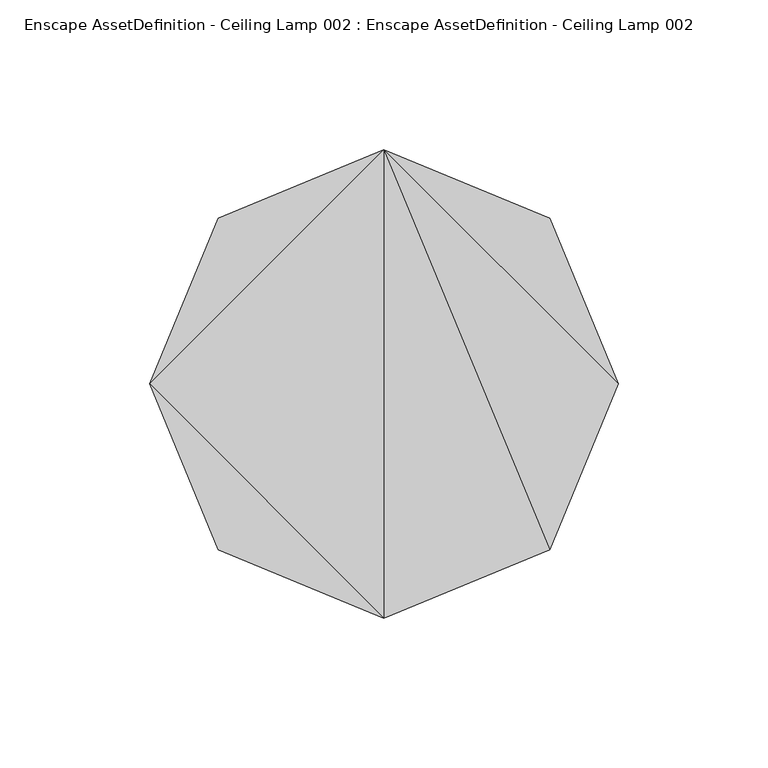
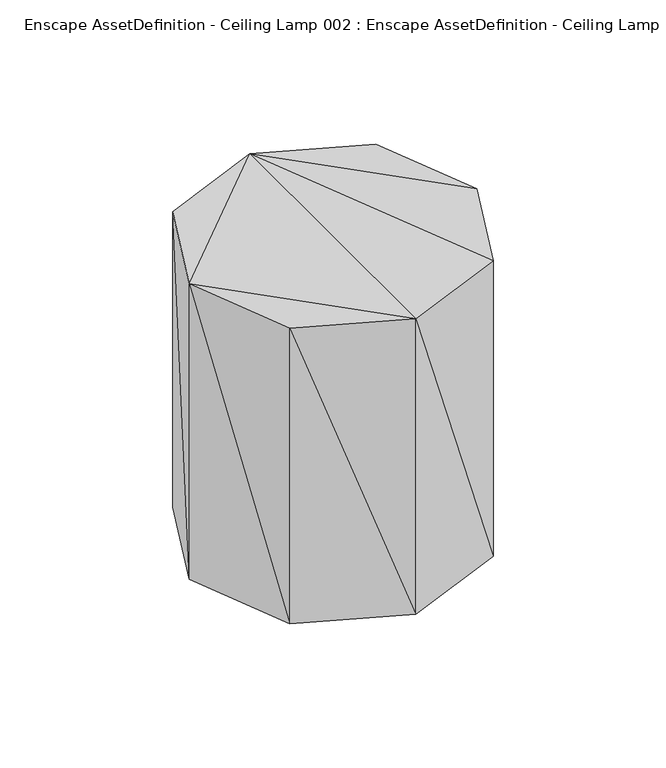
"""IFC4 building model written with IfcOpenShell, lengths in millimetres: geographic element geometry, Enscape AssetDefinition - Ceiling Lamp 002 : Enscape AssetDefinition - Ceiling Lamp 002."""

from ifc_helpers import new_model, si_unit, origin, place, context, project, spatial, faceted_brep, source, transform, mapped, element, save


def enscape_assetdefinition_ceiling_lamp_002_enscape_ece63965(model_context):
    return source(origin(), model_context, "Body", "Brep", [
        faceted_brep([(-78.1945959, 0.0, -170.0000018), (0.0, -78.1945959, -170.0000018), (-55.2917272, -55.2917272, -170.0000018), (-55.2917272, -55.2917272, 0.0), (55.2917272, -55.2917272, -170.0000018), (0.0, -78.1945959, 0.0), (-78.1945959, 0.0, 0.0), (0.0, 78.1945959, 0.0), (55.2917272, -55.2917272, 0.0), (78.1945959, 0.0, -170.0000018), (78.1945959, 0.0, 0.0), (55.2917272, 55.2917272, -170.0000018), (-55.2917272, 55.2917272, -170.0000018), (0.0, 78.1945959, -170.0000018), (55.2917272, 55.2917272, 0.0), (-55.2917272, 55.2917272, 0.0)], [[[0, 1, 2]], [[2, 1, 3]], [[1, 4, 5]], [[0, 4, 1]], [[3, 1, 5]], [[0, 2, 6]], [[6, 2, 3]], [[5, 6, 3]], [[5, 7, 6]], [[7, 5, 8]], [[5, 4, 8]], [[4, 9, 8]], [[0, 9, 4]], [[7, 8, 10]], [[8, 9, 10]], [[9, 11, 10]], [[9, 0, 12]], [[9, 12, 13]], [[9, 13, 11]], [[7, 10, 14]], [[10, 11, 14]], [[11, 13, 14]], [[13, 12, 7]], [[14, 13, 7]], [[6, 7, 15]], [[7, 12, 15]], [[15, 0, 6]], [[12, 0, 15]]]),
    ])


if __name__ == "__main__":
    model = new_model("IFC4")
    model_context = context("Model", 3, world=origin())
    ifc_project = project(units=[si_unit("LENGTHUNIT", "METRE", prefix="MILLI")], contexts=[model_context])
    site = spatial("IfcSite", under=ifc_project)
    building = spatial("IfcBuilding", under=site)
    placement = place(None, origin())
    enscape_assetdefinition_ceiling_lamp_002_enscape_shape = enscape_assetdefinition_ceiling_lamp_002_enscape_ece63965(model_context)
    element("IfcGeographicElement", 1, ObjectType="Enscape AssetDefinition - Ceiling Lamp 002 : Enscape AssetDefinition - Ceiling Lamp 002", at=placement, inside=building, context=model_context, shape_type="MappedRepresentation", body=[
        mapped(enscape_assetdefinition_ceiling_lamp_002_enscape_shape, transform((0.0, 0.0, 0.0), x_axis=(1.0, 0.0, 0.0), y_axis=(0.0, 1.0, 0.0), z_axis=(0.0, 0.0, 1.0))),
    ])
    save(model, "model.ifc")

# Revit data of these elements
# Type "Enscape AssetDefinition - Ceiling Lamp 002 : Enscape AssetDefinition - Ceiling Lamp 002"
#   EnscapeAssetSource = "REMOTE"
#   EnscapeAssetId = "d2986385-ef04-40b6-b069-b70673c39d02"
#   EnscapeNativeAssetHeight = 0 mm
#   Height = 0
#   Default Elevation = 0
